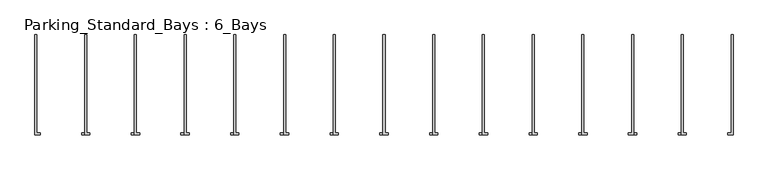
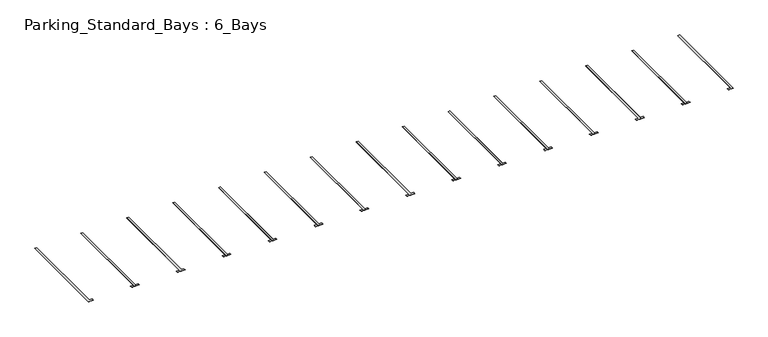
"""IFC4 building model written with IfcOpenShell, lengths in millimetres: proxy geometry, Parking_Standard_Bays : 6_Bays."""

import ifcopenshell
import ifcopenshell.guid

model = None  # the IFC model being written
_history = None  # IfcOwnerHistory: only IFC2X3 demands one
_inside = {}  # id of a spatial element -> (the spatial element, [elements in it])
_under = {}  # id of a project, library or spatial element -> (it, [spatial elements below it])
_declared = {}  # id of a project -> (the project, [libraries it declares])
_typed = {}  # id of a type object -> (the type object, [elements of that type])
_made_of = {}  # id of a material, layer set ... -> (it, [elements and type objects made of it])


def new_model(schema):
    """Start an empty IFC model of exactly this schema.

    Asked for "IFC4X3", IfcOpenShell would pick the latest addendum, in which some entities
    have other attributes; the version numbers below select the first issue.
    IFC2X3 requires an IfcOwnerHistory on every rooted entity: one is made here for all.
    """
    global model, _history
    if schema == "IFC4X3":
        model = ifcopenshell.file(schema_version=(4, 3, 0, 0))
    else:
        model = ifcopenshell.file(schema=schema)
    _inside.clear()
    _under.clear()
    _declared.clear()
    _typed.clear()
    _made_of.clear()
    _history = None
    if model.schema == "IFC2X3":
        org = make("IfcOrganization", Name="unknown")
        user = make(
            "IfcPersonAndOrganization",
            ThePerson=make("IfcPerson", FamilyName="unknown"),
            TheOrganization=org,
        )
        app = make(
            "IfcApplication",
            ApplicationDeveloper=org,
            Version="unknown",
            ApplicationFullName="unknown",
            ApplicationIdentifier="unknown",
        )
        _history = make(
            "IfcOwnerHistory",
            OwningUser=user,
            OwningApplication=app,
            ChangeAction="ADDED",
            CreationDate=0,
        )
    return model


def make(cls, **values):
    """One entity of the class cls with the attributes given. An attribute that is None is left unset."""
    return model.create_entity(
        cls, **{name: value for name, value in values.items() if value is not None}
    )


def rooted(cls, **values):
    """An entity with a GlobalId (a new one), such as an element, a storey or a relation."""
    return make(cls, GlobalId=ifcopenshell.guid.new(), OwnerHistory=_history, **values)


def si_unit(unit_type, name, prefix=None):
    """IfcSIUnit, for example si_unit("LENGTHUNIT", "METRE", prefix="MILLI")."""
    return make("IfcSIUnit", UnitType=unit_type, Prefix=prefix, Name=name)


def assignment(units):
    """IfcUnitAssignment: the units of a project."""
    return None if units is None else make("IfcUnitAssignment", Units=units)


def point(xyz):
    """IfcCartesianPoint."""
    return None if xyz is None else make("IfcCartesianPoint", Coordinates=xyz)


def direction(xyz):
    """IfcDirection."""
    return None if xyz is None else make("IfcDirection", DirectionRatios=xyz)


def frame(location, z_axis=None, x_axis=None):
    """IfcAxis2Placement3D, a coordinate frame: its origin and axes. An axis left out is left unset."""
    return make(
        "IfcAxis2Placement3D",
        Location=point(location),
        Axis=direction(z_axis),
        RefDirection=direction(x_axis),
    )


def origin():
    """The frame at (0, 0, 0) with its axes left unset."""
    return frame((0.0, 0.0, 0.0))


def origin_with_axes():
    """The frame at (0, 0, 0) with the z axis (0, 0, 1) and the x axis (1, 0, 0) written out."""
    return frame((0.0, 0.0, 0.0), z_axis=(0.0, 0.0, 1.0), x_axis=(1.0, 0.0, 0.0))


def place(relative_to, where):
    """IfcLocalPlacement: puts the frame where relative to a parent placement (None: the world)."""
    return make(
        "IfcLocalPlacement", PlacementRelTo=relative_to, RelativePlacement=where
    )


def context(
    kind, dimensions, precision=None, world=None, true_north=None, identifier=None
):
    """IfcGeometricRepresentationContext, for example the 3D "Model" context."""
    return make(
        "IfcGeometricRepresentationContext",
        ContextIdentifier=identifier,
        ContextType=kind,
        CoordinateSpaceDimension=dimensions,
        Precision=precision,
        WorldCoordinateSystem=world,
        TrueNorth=true_north,
    )


def project(units=None, contexts=None):
    """IfcProject with its units and contexts."""
    return rooted(
        "IfcProject",
        Name="project",
        RepresentationContexts=contexts,
        UnitsInContext=assignment(units),
    )


def spatial(cls, under=None, at=None, **own):
    """A site, building, storey or space (cls), placed at a placement, below another one or the project."""
    s = rooted(cls, ObjectPlacement=at, **own)
    if under is not None:
        _under.setdefault(under.id(), (under, []))[1].append(s)
    return s


def polyline(points):
    """IfcPolyline through the points."""
    return make("IfcPolyline", Points=[point(p) for p in points])


def outline(outer, holes=None, kind="AREA"):
    """IfcArbitraryClosedProfileDef: a profile drawn as a closed curve; with holes, ...WithVoids."""
    if holes is None:
        return make("IfcArbitraryClosedProfileDef", ProfileType=kind, OuterCurve=outer)
    return make(
        "IfcArbitraryProfileDefWithVoids",
        ProfileType=kind,
        OuterCurve=outer,
        InnerCurves=holes,
    )


def extrude(swept, where, along, depth):
    """IfcExtrudedAreaSolid: the profile swept, set in the frame where, extruded along a direction by depth."""
    return make(
        "IfcExtrudedAreaSolid",
        SweptArea=swept,
        Position=where,
        ExtrudedDirection=direction(along),
        Depth=depth,
    )


def shape(context_of_items, identifier, shape_type, items):
    """IfcShapeRepresentation: the items that make up one representation, for example the "Body"."""
    return make(
        "IfcShapeRepresentation",
        ContextOfItems=context_of_items,
        RepresentationIdentifier=identifier,
        RepresentationType=shape_type,
        Items=items,
    )


def source(mapping_origin, context_of_items, identifier, shape_type, items):
    """IfcRepresentationMap: a shape defined once, which mapped items show again and again."""
    return make(
        "IfcRepresentationMap",
        MappingOrigin=mapping_origin,
        MappedRepresentation=shape(context_of_items, identifier, shape_type, items),
    )


def transform(
    local_origin,
    x_axis=None,
    y_axis=None,
    z_axis=None,
    scale=None,
    scale2=None,
    scale3=None,
    uniform=True,
):
    """IfcCartesianTransformationOperator3D, or its non-uniform kind. x_axis, y_axis, z_axis: its Axis1, 2, 3."""
    if uniform:
        return make(
            "IfcCartesianTransformationOperator3D",
            Axis1=direction(x_axis),
            Axis2=direction(y_axis),
            LocalOrigin=point(local_origin),
            Scale=scale,
            Axis3=direction(z_axis),
        )
    return make(
        "IfcCartesianTransformationOperator3DnonUniform",
        Axis1=direction(x_axis),
        Axis2=direction(y_axis),
        LocalOrigin=point(local_origin),
        Scale=scale,
        Axis3=direction(z_axis),
        Scale2=scale2,
        Scale3=scale3,
    )


def mapped(mapping_source, mapping_target):
    """IfcMappedItem: shows the shape of a source again, moved by a transform."""
    return make(
        "IfcMappedItem", MappingSource=mapping_source, MappingTarget=mapping_target
    )


def made_of(thing, what):
    """Note that an element or type object is made of a material, layer set ...; save() writes the relation."""
    if what is not None:
        _made_of.setdefault(what.id(), (what, []))[1].append(thing)
    return thing


def element(
    cls,
    number,
    at=None,
    inside=None,
    cuts=None,
    type_object=None,
    material=None,
    context=None,
    identifier="Body",
    shape_type=None,
    held_by="IfcProductDefinitionShape",
    body=None,
    shapes=None,
    **own,
):
    """One element of the class cls, such as IfcWall. Its Tag is "e" and its number.

    at: its placement. inside: the storey or other place that contains it. cuts: it is an
    opening in that element (IfcRelVoidsElement). A single representation is given by context,
    identifier, shape_type and body (its items); several are given by shapes. held_by: the class
    of the entity that holds the representations. save() writes the other relations.
    """
    e = rooted(cls, Tag="e%d" % number, ObjectPlacement=at, **own)
    if body is not None:
        shapes = [shape(context, identifier, shape_type, body)]
    if shapes is not None:
        e.Representation = make(held_by, Representations=shapes)
    if inside is not None:
        _inside.setdefault(inside.id(), (inside, []))[1].append(e)
    if cuts is not None:
        rooted(
            "IfcRelVoidsElement", RelatingBuildingElement=cuts, RelatedOpeningElement=e
        )
    if type_object is not None:
        _typed.setdefault(type_object.id(), (type_object, []))[1].append(e)
    return made_of(e, material)


def aggregate(whole, parts):
    """IfcRelAggregates: a whole, such as a stair, and the parts it consists of."""
    return rooted("IfcRelAggregates", RelatingObject=whole, RelatedObjects=parts)


def save(model, path):
    """Write the relations noted so far, then the file.

    IfcRelAggregates (storeys below a building ...), IfcRelContainedInSpatialStructure (elements
    in a storey), IfcRelDefinesByType, IfcRelAssociatesMaterial and IfcRelDeclares: one each for
    every whole, place, type object, material and project.
    """
    for whole, parts in _under.values():
        aggregate(whole, parts)
    for where, things in _inside.values():
        rooted(
            "IfcRelContainedInSpatialStructure",
            RelatedElements=things,
            RelatingStructure=where,
        )
    for kind, things in _typed.values():
        rooted("IfcRelDefinesByType", RelatedObjects=things, RelatingType=kind)
    for what, things in _made_of.values():
        rooted("IfcRelAssociatesMaterial", RelatedObjects=things, RelatingMaterial=what)
    for by, libraries in _declared.values():
        rooted("IfcRelDeclares", RelatingContext=by, RelatedDefinitions=libraries)
    model.write(path)


def parking_standard_bays_6_bays_7b2c0127(model_context):
    return source(origin(), model_context, "Body", "SweptSolid", [
        extrude(outline(polyline([(28750.0, 0.0), (28850.0, 0.0), (28850.0, -4850.0), (28600.0, -4850.0), (28600.0, -4750.0), (28750.0, -4750.0), (28750.0, 0.0)])), origin_with_axes(), (0.0, 0.0, 1.0), 3.175),
        extrude(outline(polyline([(26350.0, 0.0), (26450.0, 0.0), (26450.0, -4750.0), (26600.0, -4750.0), (26600.0, -4850.0), (26350.0, -4850.0), (26350.0, 0.0)])), origin_with_axes(), (0.0, 0.0, 1.0), 3.175),
        extrude(outline(polyline([(26350.0, 0.0), (26450.0, 0.0), (26450.0, -4850.0), (26200.0, -4850.0), (26200.0, -4750.0), (26350.0, -4750.0), (26350.0, 0.0)])), origin_with_axes(), (0.0, 0.0, 1.0), 3.175),
        extrude(outline(polyline([(23950.0, 0.0), (24050.0, 0.0), (24050.0, -4750.0), (24200.0, -4750.0), (24200.0, -4850.0), (23950.0, -4850.0), (23950.0, 0.0)])), origin_with_axes(), (0.0, 0.0, 1.0), 3.175),
        extrude(outline(polyline([(23950.0, 0.0), (24050.0, 0.0), (24050.0, -4850.0), (23800.0, -4850.0), (23800.0, -4750.0), (23950.0, -4750.0), (23950.0, 0.0)])), origin_with_axes(), (0.0, 0.0, 1.0), 3.175),
        extrude(outline(polyline([(21550.0, 0.0), (21650.0, 0.0), (21650.0, -4750.0), (21800.0, -4750.0), (21800.0, -4850.0), (21550.0, -4850.0), (21550.0, 0.0)])), origin_with_axes(), (0.0, 0.0, 1.0), 3.175),
        extrude(outline(polyline([(21550.0, 0.0), (21650.0, 0.0), (21650.0, -4850.0), (21400.0, -4850.0), (21400.0, -4750.0), (21550.0, -4750.0), (21550.0, 0.0)])), origin_with_axes(), (0.0, 0.0, 1.0), 3.175),
        extrude(outline(polyline([(19150.0, 0.0), (19250.0, 0.0), (19250.0, -4750.0), (19400.0, -4750.0), (19400.0, -4850.0), (19150.0, -4850.0), (19150.0, 0.0)])), origin_with_axes(), (0.0, 0.0, 1.0), 3.175),
        extrude(outline(polyline([(19150.0, 0.0), (19250.0, 0.0), (19250.0, -4850.0), (19000.0, -4850.0), (19000.0, -4750.0), (19150.0, -4750.0), (19150.0, 0.0)])), origin_with_axes(), (0.0, 0.0, 1.0), 3.175),
        extrude(outline(polyline([(16750.0, 0.0), (16850.0, 0.0), (16850.0, -4750.0), (17000.0, -4750.0), (17000.0, -4850.0), (16750.0, -4850.0), (16750.0, 0.0)])), origin_with_axes(), (0.0, 0.0, 1.0), 3.175),
        extrude(outline(polyline([(16750.0, 0.0), (16850.0, 0.0), (16850.0, -4850.0), (16600.0, -4850.0), (16600.0, -4750.0), (16750.0, -4750.0), (16750.0, 0.0)])), origin_with_axes(), (0.0, 0.0, 1.0), 3.175),
        extrude(outline(polyline([(14350.0, 0.0), (14450.0, 0.0), (14450.0, -4750.0), (14600.0, -4750.0), (14600.0, -4850.0), (14350.0, -4850.0), (14350.0, 0.0)])), origin_with_axes(), (0.0, 0.0, 1.0), 3.175),
        extrude(outline(polyline([(14350.0, 0.0), (14450.0, 0.0), (14450.0, -4850.0), (14200.0, -4850.0), (14200.0, -4750.0), (14350.0, -4750.0), (14350.0, 0.0)])), origin_with_axes(), (0.0, 0.0, 1.0), 3.175),
        extrude(outline(polyline([(11950.0, 0.0), (12050.0, 0.0), (12050.0, -4750.0), (12200.0, -4750.0), (12200.0, -4850.0), (11950.0, -4850.0), (11950.0, 0.0)])), origin_with_axes(), (0.0, 0.0, 1.0), 3.175),
        extrude(outline(polyline([(11950.0, 0.0), (12050.0, 0.0), (12050.0, -4850.0), (11800.0, -4850.0), (11800.0, -4750.0), (11950.0, -4750.0), (11950.0, 0.0)])), origin_with_axes(), (0.0, 0.0, 1.0), 3.175),
        extrude(outline(polyline([(9550.0, 0.0), (9650.0, 0.0), (9650.0, -4750.0), (9800.0, -4750.0), (9800.0, -4850.0), (9550.0, -4850.0), (9550.0, 0.0)])), origin_with_axes(), (0.0, 0.0, 1.0), 3.175),
        extrude(outline(polyline([(33550.0, 0.0), (33650.0, 0.0), (33650.0, -4850.0), (33400.0, -4850.0), (33400.0, -4750.0), (33550.0, -4750.0), (33550.0, 0.0)])), origin_with_axes(), (0.0, 0.0, 1.0), 3.175),
        extrude(outline(polyline([(31150.0, 0.0), (31250.0, 0.0), (31250.0, -4750.0), (31400.0, -4750.0), (31400.0, -4850.0), (31150.0, -4850.0), (31150.0, 0.0)])), origin_with_axes(), (0.0, 0.0, 1.0), 3.175),
        extrude(outline(polyline([(9550.0, 0.0), (9650.0, 0.0), (9650.0, -4850.0), (9400.0, -4850.0), (9400.0, -4750.0), (9550.0, -4750.0), (9550.0, 0.0)])), origin_with_axes(), (0.0, 0.0, 1.0), 3.175),
        extrude(outline(polyline([(7150.0, 0.0), (7250.0, 0.0), (7250.0, -4750.0), (7400.0, -4750.0), (7400.0, -4850.0), (7150.0, -4850.0), (7150.0, 0.0)])), origin_with_axes(), (0.0, 0.0, 1.0), 3.175),
        extrude(outline(polyline([(7150.0, 0.0), (7250.0, 0.0), (7250.0, -4850.0), (7000.0, -4850.0), (7000.0, -4750.0), (7150.0, -4750.0), (7150.0, 0.0)])), origin_with_axes(), (0.0, 0.0, 1.0), 3.175),
        extrude(outline(polyline([(4750.0, 0.0), (4850.0, 0.0), (4850.0, -4750.0), (5000.0, -4750.0), (5000.0, -4850.0), (4750.0, -4850.0), (4750.0, 0.0)])), origin_with_axes(), (0.0, 0.0, 1.0), 3.175),
        extrude(outline(polyline([(4750.0, 0.0), (4850.0, 0.0), (4850.0, -4850.0), (4600.0, -4850.0), (4600.0, -4750.0), (4750.0, -4750.0), (4750.0, 0.0)])), origin_with_axes(), (0.0, 0.0, 1.0), 3.175),
        extrude(outline(polyline([(2350.0, 0.0), (2450.0, 0.0), (2450.0, -4750.0), (2600.0, -4750.0), (2600.0, -4850.0), (2350.0, -4850.0), (2350.0, 0.0)])), origin_with_axes(), (0.0, 0.0, 1.0), 3.175),
        extrude(outline(polyline([(31150.0, 0.0), (31250.0, 0.0), (31250.0, -4850.0), (31000.0, -4850.0), (31000.0, -4750.0), (31150.0, -4750.0), (31150.0, 0.0)])), origin_with_axes(), (0.0, 0.0, 1.0), 3.175),
        extrude(outline(polyline([(28750.0, 0.0), (28850.0, 0.0), (28850.0, -4750.0), (29000.0, -4750.0), (29000.0, -4850.0), (28750.0, -4850.0), (28750.0, 0.0)])), origin_with_axes(), (0.0, 0.0, 1.0), 3.175),
        extrude(outline(polyline([(2350.0, 0.0), (2450.0, 0.0), (2450.0, -4850.0), (2200.0, -4850.0), (2200.0, -4750.0), (2350.0, -4750.0), (2350.0, 0.0)])), origin_with_axes(), (0.0, 0.0, 1.0), 3.175),
        extrude(outline(polyline([(-50.0, 0.0), (50.0, 0.0), (50.0, -4750.0), (200.0, -4750.0), (200.0, -4850.0), (-50.0, -4850.0), (-50.0, 0.0)])), origin_with_axes(), (0.0, 0.0, 1.0), 3.175),
    ])


if __name__ == "__main__":
    model = new_model("IFC4")
    model_context = context("Model", 3, world=origin())
    ifc_project = project(units=[si_unit("LENGTHUNIT", "METRE", prefix="MILLI")], contexts=[model_context])
    site = spatial("IfcSite", under=ifc_project)
    building = spatial("IfcBuilding", under=site)
    placement = place(None, origin())
    parking_standard_bays_6_bays_shape = parking_standard_bays_6_bays_7b2c0127(model_context)
    element("IfcBuildingElementProxy", 1, Name="Parking_Standard_Bays : 6_Bays", ObjectType="Parking_Standard_Bays : 6_Bays", at=placement, inside=building, context=model_context, shape_type="MappedRepresentation", body=[
        mapped(parking_standard_bays_6_bays_shape, transform((0.0, 0.0, 0.0), x_axis=(1.0, 0.0, 0.0), y_axis=(0.0, 1.0, 0.0), z_axis=(0.0, 0.0, 1.0))),
    ])
    save(model, "model.ifc")

# Revit data of these elements
# Type "Parking_Standard_Bays : 6_Bays"
#   Keynote = "Q22/185"
#   Length [instance default] = 14400 mm
#   Bay Width = 2400 mm
#   Bay Length = 4800 mm
#   No of Bays in Array [instance default] = 5
#   No of Bays [instance default] = 6
#   Material - White Lining = Paint - White Lining
# Element 1 (IfcBuildingElementProxy, "Parking_Standard_Bays : 6_Bays")
#   Length = 33600 mm
#   No of Bays in Array = 13
#   No of Bays = 14
#   Materials on its faces: "Paint - White Lining"
# Materials
#   "Paint - White Lining": class "Paint", colour RGB 239 247 247, transparency 0, Cost = 0
